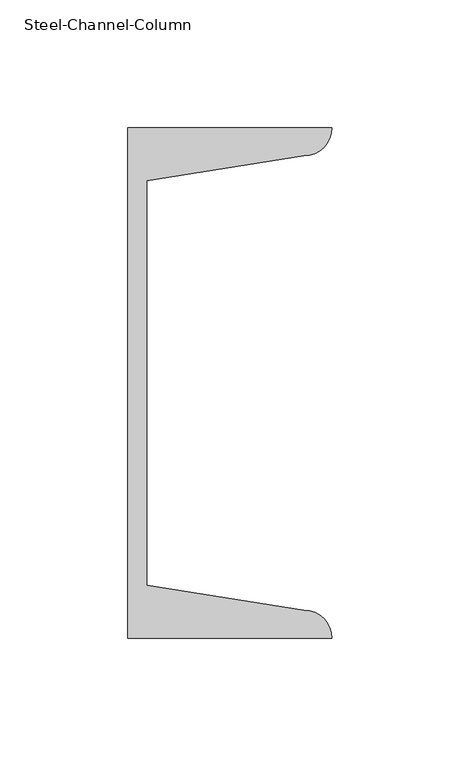
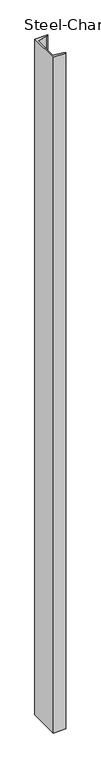
"""IFC4 building model written with IfcOpenShell, lengths in millimetres: column geometry, Steel-Channel-Column : CL126_C-200×80x7.5x11."""

from ifc_helpers import new_model, si_unit, point, frame_2d, origin, origin_with_axes, place, context, project, spatial, polyline, circle_curve, trimmed, segment, composite_curve, outline, extrude, source, transform, mapped, element, save


def steel_channel_column_de75dd10(model_context):
    return source(origin(), model_context, "Body", "SweptSolid", [
        extrude(outline(composite_curve([segment(polyline([(-22.1, 100.0), (57.9, 100.0)]), True, "CONTINUOUS"), segment(trimmed(circle_curve(frame_2d((46.9, 100.0)), 11.0), [point((57.9, 100.0))], [point((46.9, 89.0))], False, "CARTESIAN"), True, "CONTINUOUS"), segment(polyline([(46.9, 89.0), (-14.6, 79.2593569), (-14.6, -79.2593569), (46.9, -89.0)]), True, "CONTINUOUS"), segment(trimmed(circle_curve(frame_2d((46.9, -100.0)), 11.0), [point((46.9, -89.0))], [point((57.9, -100.0))], False, "CARTESIAN"), True, "CONTINUOUS"), segment(polyline([(57.9, -100.0), (-22.1, -100.0), (-22.1, 100.0)]), True, "CONTINUOUS")], self_intersect=False)), origin_with_axes(), (0.0, 0.0, 1.0), 4500.0),
    ])


if __name__ == "__main__":
    model = new_model("IFC4")
    model_context = context("Model", 3, world=origin())
    ifc_project = project(units=[si_unit("LENGTHUNIT", "METRE", prefix="MILLI")], contexts=[model_context])
    site = spatial("IfcSite", under=ifc_project)
    building = spatial("IfcBuilding", under=site)
    placement = place(None, origin())
    steel_channel_column_shape = steel_channel_column_de75dd10(model_context)
    element("IfcColumn", 1, ObjectType="Steel-Channel-Column : CL126_C-200×80x7.5x11", at=placement, inside=building, context=model_context, shape_type="MappedRepresentation", body=[
        mapped(steel_channel_column_shape, transform((0.0, 0.0, 0.0), x_axis=(1.0, 0.0, 0.0), y_axis=(0.0, 1.0, 0.0), z_axis=(0.0, 0.0, 1.0))),
    ])
    save(model, "model.ifc")

# Revit data of these elements
# Type "Steel-Channel-Column : CL126_C-200×80x7.5x11"
#   Assembly Code = "B10"
#   x = 22.1 mm
#   Surface Area = 0.705 m²/m
#   Section Area = 31.33 cm²
#   Mass per Unit Length = 24.60 kg/m
#   bf = 80 mm
#   d = 200 mm
#   tf = 11 mm
#   tw = 7.5 mm
#   hec_material4 [instance default] = none
#   hec_material3 [instance default] = none
#   hec_material2 [instance default] = none
#   hec_material1 [instance default] = none
#   Structural Material [instance default] = Steel, 45-345
# Element 1 (IfcColumn, "Steel-Channel-Column : CL126_C-200×80x7.5x11")
#   Materials on its faces: "Steel, 45-345"
# Materials
#   "Steel, 45-345": class "Metal", colour RGB 189 187 185, transparency 0, Description = "Steel 345 MPa", Cost = 0
